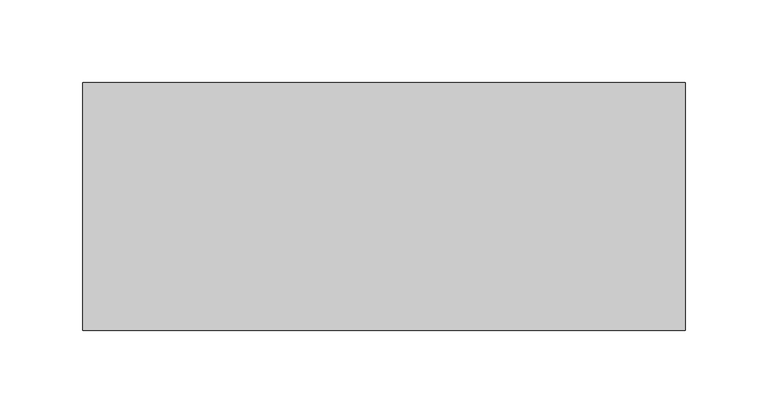
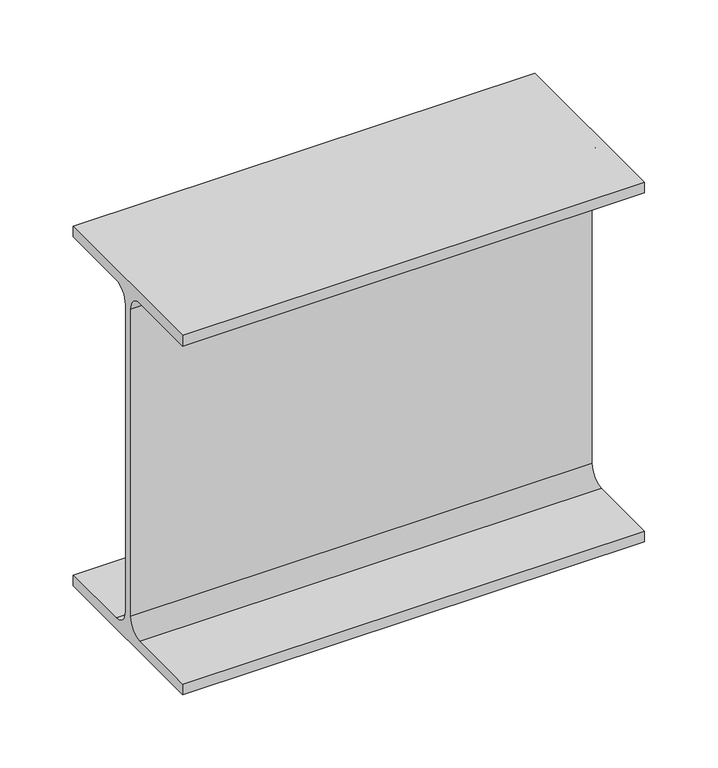
"""IFC4 building model written with IfcOpenShell, lengths in millimetres: beam geometry, 0912_Steel Framing_H-KSD3502 : H_SB_ASB_H-300x150x6.5x9."""

from ifc_helpers import new_model, si_unit, point, frame, frame_2d, origin, place, context, project, spatial, polyline, circle_curve, trimmed, segment, composite_curve, outline, extrude, source, transform, mapped, element, save


def beam_e9ed0d81(model_context):
    return source(origin(), model_context, "Body", "SweptSolid", [
        extrude(outline(composite_curve([segment(polyline([(75.0, -141.0), (75.0, -150.0), (-75.0, -150.0), (-75.0, -141.0), (-16.25, -141.0)]), True, "CONTINUOUS"), segment(trimmed(circle_curve(frame_2d((-16.25, -128.0)), 13.0), [point((-16.25, -141.0))], [point((-3.25, -128.0))], True, "CARTESIAN"), True, "CONTINUOUS"), segment(polyline([(-3.25, -128.0), (-3.25, 128.0)]), True, "CONTINUOUS"), segment(trimmed(circle_curve(frame_2d((-16.25, 128.0)), 13.0), [point((-3.25, 128.0))], [point((-16.25, 141.0))], True, "CARTESIAN"), True, "CONTINUOUS"), segment(polyline([(-16.25, 141.0), (-75.0, 141.0), (-75.0, 150.0), (75.0, 150.0), (75.0, 141.0), (16.25, 141.0)]), True, "CONTINUOUS"), segment(trimmed(circle_curve(frame_2d((16.25, 128.0)), 13.0), [point((16.25, 141.0))], [point((3.25, 128.0))], True, "CARTESIAN"), True, "CONTINUOUS"), segment(polyline([(3.25, 128.0), (3.25, -128.0)]), True, "CONTINUOUS"), segment(trimmed(circle_curve(frame_2d((16.25, -128.0)), 13.0), [point((3.25, -128.0))], [point((16.25, -141.0))], True, "CARTESIAN"), True, "CONTINUOUS"), segment(polyline([(16.25, -141.0), (75.0, -141.0)]), True, "CONTINUOUS")], self_intersect=False)), frame((-282.3, 0.0, 0.0), z_axis=(1.0, 0.0, 0.0), x_axis=(0.0, 1.0, 0.0)), (0.0, 0.0, 1.0), 364.6),
    ])


if __name__ == "__main__":
    model = new_model("IFC4")
    model_context = context("Model", 3, world=origin())
    ifc_project = project(units=[si_unit("LENGTHUNIT", "METRE", prefix="MILLI")], contexts=[model_context])
    site = spatial("IfcSite", under=ifc_project)
    building = spatial("IfcBuilding", under=site)
    placement = place(None, origin())
    beam_shape = beam_e9ed0d81(model_context)
    element("IfcBeam", 1, ObjectType="0912_Steel Framing_H-KSD3502 : H_SB_ASB_H-300x150x6.5x9", at=placement, inside=building, context=model_context, shape_type="MappedRepresentation", body=[
        mapped(beam_shape, transform((0.0, 0.0, 0.0), x_axis=(1.0, 0.0, 0.0), y_axis=(0.0, 1.0, 0.0), z_axis=(0.0, 0.0, 1.0))),
    ])
    save(model, "model.ifc")

# Revit data of these elements
# Type "0912_Steel Framing_H-KSD3502 : H_SB_ASB_H-300x150x6.5x9"
#   H_WM Code_1 = "S01AA002-00001 | Main Steel Structure Fabrication Work | Shelter/Building | Medium Steel - Standard (90KG/M>Weight≥30KG/M) | Material: (   )"
#   H_WM Code_2 = "S03AA028-00001 | Main Steel Structure Erection Work | Shelter/Building | Medium Steel (90KG/M>Weight≥30KG/M) | Material: (   )"
#   H_WM Code_3 = "S01AA010-00001 | Main Steel Structure Fabrication Work | Shelter/Building | Steel Painting/Coating | for Non-Fireproofed Steel Surface, Surface Preparation, Primer, Second & Final Coat | Material: (   )"
#   H_Q'ty Cal Type Tag = "SB-Q2"
#   Width = 15.0 cm
#   Web Thickness = 0.65 cm
#   Web Fillet = 1.3 cm
#   Warping Constant = 107000.0 cm⁶
#   W = 0
#   Torsional Moment of Inertia = 9.9539 cm⁴
#   Section Area = 46.78 cm²
#   Plastic Modulus weak axis = 105.0 cm³
#   Plastic Modulus strong axis = 542.0 cm³
#   Perimeter = 1.17 m²/m
#   Nominal Weight = 36.70 kgf/m
#   Moment of Inertia weak axis = 508.00 cm⁴
#   Moment of Inertia strong axis = 7210.00 cm⁴
#   Height = 30.0 cm
#   Flange Thickness = 0.9 cm
#   Elastic Modulus weak axis = 67.7 cm³
#   Elastic Modulus strong axis = 481.0 cm³
#   Centroid Vertical = 15.0 cm
#   Centroid Horizontal = 7.5 cm
#   Ix = 72100000
#   Length [instance default] = 1.5240 m
#   Zx = 542000
#   b = 0.1500 m
#   h = 0.3000 m
#   r = 0.0130 m
#   s = 0.0065 m
#   t = 0.0090 m
#   A = 0.004678 m²
#   Structural Material [instance default] = Steel, 45-345
#   Assembly Code = ""
# Element 1 (IfcBeam, "0912_Steel Framing_H-KSD3502 : H_SB_ASB_H-300x150x6.5x9")
#   Structural Material = none
# Materials
#   "Steel, 45-345": class "Metal", colour RGB 189 187 185, transparency 0, Description = "Steel 345 MPa", Cost = 0
